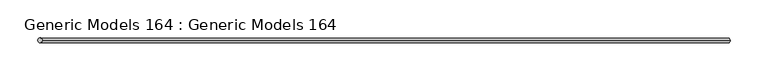
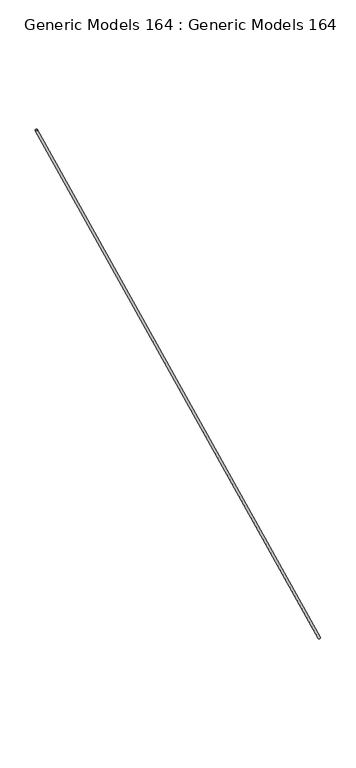
"""IFC4 building model written with IfcOpenShell, lengths in millimetres: proxy geometry, Generic Models 164 : Generic Models 164."""

import ifcopenshell
import ifcopenshell.guid

model = None  # the IFC model being written
_history = None  # IfcOwnerHistory: only IFC2X3 demands one
_inside = {}  # id of a spatial element -> (the spatial element, [elements in it])
_under = {}  # id of a project, library or spatial element -> (it, [spatial elements below it])
_declared = {}  # id of a project -> (the project, [libraries it declares])
_typed = {}  # id of a type object -> (the type object, [elements of that type])
_made_of = {}  # id of a material, layer set ... -> (it, [elements and type objects made of it])


def new_model(schema):
    """Start an empty IFC model of exactly this schema.

    Asked for "IFC4X3", IfcOpenShell would pick the latest addendum, in which some entities
    have other attributes; the version numbers below select the first issue.
    IFC2X3 requires an IfcOwnerHistory on every rooted entity: one is made here for all.
    """
    global model, _history
    if schema == "IFC4X3":
        model = ifcopenshell.file(schema_version=(4, 3, 0, 0))
    else:
        model = ifcopenshell.file(schema=schema)
    _inside.clear()
    _under.clear()
    _declared.clear()
    _typed.clear()
    _made_of.clear()
    _history = None
    if model.schema == "IFC2X3":
        org = make("IfcOrganization", Name="unknown")
        user = make(
            "IfcPersonAndOrganization",
            ThePerson=make("IfcPerson", FamilyName="unknown"),
            TheOrganization=org,
        )
        app = make(
            "IfcApplication",
            ApplicationDeveloper=org,
            Version="unknown",
            ApplicationFullName="unknown",
            ApplicationIdentifier="unknown",
        )
        _history = make(
            "IfcOwnerHistory",
            OwningUser=user,
            OwningApplication=app,
            ChangeAction="ADDED",
            CreationDate=0,
        )
    return model


def make(cls, **values):
    """One entity of the class cls with the attributes given. An attribute that is None is left unset."""
    return model.create_entity(
        cls, **{name: value for name, value in values.items() if value is not None}
    )


def rooted(cls, **values):
    """An entity with a GlobalId (a new one), such as an element, a storey or a relation."""
    return make(cls, GlobalId=ifcopenshell.guid.new(), OwnerHistory=_history, **values)


def si_unit(unit_type, name, prefix=None):
    """IfcSIUnit, for example si_unit("LENGTHUNIT", "METRE", prefix="MILLI")."""
    return make("IfcSIUnit", UnitType=unit_type, Prefix=prefix, Name=name)


def assignment(units):
    """IfcUnitAssignment: the units of a project."""
    return None if units is None else make("IfcUnitAssignment", Units=units)


def point(xyz):
    """IfcCartesianPoint."""
    return None if xyz is None else make("IfcCartesianPoint", Coordinates=xyz)


def direction(xyz):
    """IfcDirection."""
    return None if xyz is None else make("IfcDirection", DirectionRatios=xyz)


def frame(location, z_axis=None, x_axis=None):
    """IfcAxis2Placement3D, a coordinate frame: its origin and axes. An axis left out is left unset."""
    return make(
        "IfcAxis2Placement3D",
        Location=point(location),
        Axis=direction(z_axis),
        RefDirection=direction(x_axis),
    )


def frame_2d(location, x_axis=None):
    """IfcAxis2Placement2D, a coordinate frame in the plane: its origin and x axis."""
    return make(
        "IfcAxis2Placement2D", Location=point(location), RefDirection=direction(x_axis)
    )


def origin():
    """The frame at (0, 0, 0) with its axes left unset."""
    return frame((0.0, 0.0, 0.0))


def place(relative_to, where):
    """IfcLocalPlacement: puts the frame where relative to a parent placement (None: the world)."""
    return make(
        "IfcLocalPlacement", PlacementRelTo=relative_to, RelativePlacement=where
    )


def context(
    kind, dimensions, precision=None, world=None, true_north=None, identifier=None
):
    """IfcGeometricRepresentationContext, for example the 3D "Model" context."""
    return make(
        "IfcGeometricRepresentationContext",
        ContextIdentifier=identifier,
        ContextType=kind,
        CoordinateSpaceDimension=dimensions,
        Precision=precision,
        WorldCoordinateSystem=world,
        TrueNorth=true_north,
    )


def project(units=None, contexts=None):
    """IfcProject with its units and contexts."""
    return rooted(
        "IfcProject",
        Name="project",
        RepresentationContexts=contexts,
        UnitsInContext=assignment(units),
    )


def spatial(cls, under=None, at=None, **own):
    """A site, building, storey or space (cls), placed at a placement, below another one or the project."""
    s = rooted(cls, ObjectPlacement=at, **own)
    if under is not None:
        _under.setdefault(under.id(), (under, []))[1].append(s)
    return s


def circle_curve(where, radius):
    """IfcCircle in the frame where."""
    return make("IfcCircle", Position=where, Radius=radius)


def trimmed(basis, trim1, trim2, sense, master):
    """IfcTrimmedCurve: the piece of a basis curve between two trims."""
    return make(
        "IfcTrimmedCurve",
        BasisCurve=basis,
        Trim1=trim1,
        Trim2=trim2,
        SenseAgreement=sense,
        MasterRepresentation=master,
    )


def segment(curve, same_sense, transition):
    """IfcCompositeCurveSegment."""
    return make(
        "IfcCompositeCurveSegment",
        Transition=transition,
        SameSense=same_sense,
        ParentCurve=curve,
    )


def composite_curve(segments, self_intersect=None):
    """IfcCompositeCurve: segments joined end to end."""
    return make("IfcCompositeCurve", Segments=segments, SelfIntersect=self_intersect)


def outline(outer, holes=None, kind="AREA"):
    """IfcArbitraryClosedProfileDef: a profile drawn as a closed curve; with holes, ...WithVoids."""
    if holes is None:
        return make("IfcArbitraryClosedProfileDef", ProfileType=kind, OuterCurve=outer)
    return make(
        "IfcArbitraryProfileDefWithVoids",
        ProfileType=kind,
        OuterCurve=outer,
        InnerCurves=holes,
    )


def extrude(swept, where, along, depth):
    """IfcExtrudedAreaSolid: the profile swept, set in the frame where, extruded along a direction by depth."""
    return make(
        "IfcExtrudedAreaSolid",
        SweptArea=swept,
        Position=where,
        ExtrudedDirection=direction(along),
        Depth=depth,
    )


def shape(context_of_items, identifier, shape_type, items):
    """IfcShapeRepresentation: the items that make up one representation, for example the "Body"."""
    return make(
        "IfcShapeRepresentation",
        ContextOfItems=context_of_items,
        RepresentationIdentifier=identifier,
        RepresentationType=shape_type,
        Items=items,
    )


def source(mapping_origin, context_of_items, identifier, shape_type, items):
    """IfcRepresentationMap: a shape defined once, which mapped items show again and again."""
    return make(
        "IfcRepresentationMap",
        MappingOrigin=mapping_origin,
        MappedRepresentation=shape(context_of_items, identifier, shape_type, items),
    )


def transform(
    local_origin,
    x_axis=None,
    y_axis=None,
    z_axis=None,
    scale=None,
    scale2=None,
    scale3=None,
    uniform=True,
):
    """IfcCartesianTransformationOperator3D, or its non-uniform kind. x_axis, y_axis, z_axis: its Axis1, 2, 3."""
    if uniform:
        return make(
            "IfcCartesianTransformationOperator3D",
            Axis1=direction(x_axis),
            Axis2=direction(y_axis),
            LocalOrigin=point(local_origin),
            Scale=scale,
            Axis3=direction(z_axis),
        )
    return make(
        "IfcCartesianTransformationOperator3DnonUniform",
        Axis1=direction(x_axis),
        Axis2=direction(y_axis),
        LocalOrigin=point(local_origin),
        Scale=scale,
        Axis3=direction(z_axis),
        Scale2=scale2,
        Scale3=scale3,
    )


def mapped(mapping_source, mapping_target):
    """IfcMappedItem: shows the shape of a source again, moved by a transform."""
    return make(
        "IfcMappedItem", MappingSource=mapping_source, MappingTarget=mapping_target
    )


def made_of(thing, what):
    """Note that an element or type object is made of a material, layer set ...; save() writes the relation."""
    if what is not None:
        _made_of.setdefault(what.id(), (what, []))[1].append(thing)
    return thing


def element(
    cls,
    number,
    at=None,
    inside=None,
    cuts=None,
    type_object=None,
    material=None,
    context=None,
    identifier="Body",
    shape_type=None,
    held_by="IfcProductDefinitionShape",
    body=None,
    shapes=None,
    **own,
):
    """One element of the class cls, such as IfcWall. Its Tag is "e" and its number.

    at: its placement. inside: the storey or other place that contains it. cuts: it is an
    opening in that element (IfcRelVoidsElement). A single representation is given by context,
    identifier, shape_type and body (its items); several are given by shapes. held_by: the class
    of the entity that holds the representations. save() writes the other relations.
    """
    e = rooted(cls, Tag="e%d" % number, ObjectPlacement=at, **own)
    if body is not None:
        shapes = [shape(context, identifier, shape_type, body)]
    if shapes is not None:
        e.Representation = make(held_by, Representations=shapes)
    if inside is not None:
        _inside.setdefault(inside.id(), (inside, []))[1].append(e)
    if cuts is not None:
        rooted(
            "IfcRelVoidsElement", RelatingBuildingElement=cuts, RelatedOpeningElement=e
        )
    if type_object is not None:
        _typed.setdefault(type_object.id(), (type_object, []))[1].append(e)
    return made_of(e, material)


def aggregate(whole, parts):
    """IfcRelAggregates: a whole, such as a stair, and the parts it consists of."""
    return rooted("IfcRelAggregates", RelatingObject=whole, RelatedObjects=parts)


def save(model, path):
    """Write the relations noted so far, then the file.

    IfcRelAggregates (storeys below a building ...), IfcRelContainedInSpatialStructure (elements
    in a storey), IfcRelDefinesByType, IfcRelAssociatesMaterial and IfcRelDeclares: one each for
    every whole, place, type object, material and project.
    """
    for whole, parts in _under.values():
        aggregate(whole, parts)
    for where, things in _inside.values():
        rooted(
            "IfcRelContainedInSpatialStructure",
            RelatedElements=things,
            RelatingStructure=where,
        )
    for kind, things in _typed.values():
        rooted("IfcRelDefinesByType", RelatedObjects=things, RelatingType=kind)
    for what, things in _made_of.values():
        rooted("IfcRelAssociatesMaterial", RelatedObjects=things, RelatingMaterial=what)
    for by, libraries in _declared.values():
        rooted("IfcRelDeclares", RelatingContext=by, RelatedDefinitions=libraries)
    model.write(path)


def generic_models_164_generic_models_164_470bc0f9(model_context):
    return source(origin(), model_context, "Body", "SweptSolid", [
        extrude(outline(composite_curve([segment(trimmed(circle_curve(frame_2d((0.0, -3.175)), 3.175), [point((0.0, -6.35))], [point((0.0, 0.0))], False, "CARTESIAN"), True, "CONTINUOUS"), segment(trimmed(circle_curve(frame_2d((0.0, -3.175)), 3.175), [point((0.0, 0.0))], [point((0.0, -6.35))], False, "CARTESIAN"), True, "CONTINUOUS")], self_intersect=False)), frame((34361.4578689, 41017.9182538, 266524.7126687), z_axis=(-0.40686458181291274, 0.0, 0.913488484911662), x_axis=(0.0, -1.0, 0.0)), (0.0, 0.0, 1.0), 2230.672779),
    ])


if __name__ == "__main__":
    model = new_model("IFC4")
    model_context = context("Model", 3, world=origin())
    ifc_project = project(units=[si_unit("LENGTHUNIT", "METRE", prefix="MILLI")], contexts=[model_context])
    site = spatial("IfcSite", under=ifc_project)
    building = spatial("IfcBuilding", under=site)
    placement = place(None, origin())
    generic_models_164_generic_models_164_shape = generic_models_164_generic_models_164_470bc0f9(model_context)
    element("IfcBuildingElementProxy", 1, Name="Generic Models 164 : Generic Models 164", ObjectType="Generic Models 164 : Generic Models 164", at=placement, inside=building, context=model_context, shape_type="MappedRepresentation", body=[
        mapped(generic_models_164_generic_models_164_shape, transform((0.0, 0.0, 0.0), x_axis=(1.0, 0.0, 0.0), y_axis=(0.0, 1.0, 0.0), z_axis=(0.0, 0.0, 1.0))),
    ])
    save(model, "model.ifc")

# Revit data of these elements
# Element 1 (IfcBuildingElementProxy, "Generic Models 164 : Generic Models 164")
#   Materials on its faces: "1/4\" GALV ROD - TURNBUCKLES - EYEHOOKS"
# Materials
#   "1/4\" GALV ROD - TURNBUCKLES - EYEHOOKS": class "Metal", colour RGB 199 199 199, transparency 0, Description = "Structural steel, ASTM A36 Grade B, mill finish", Cost = 0
